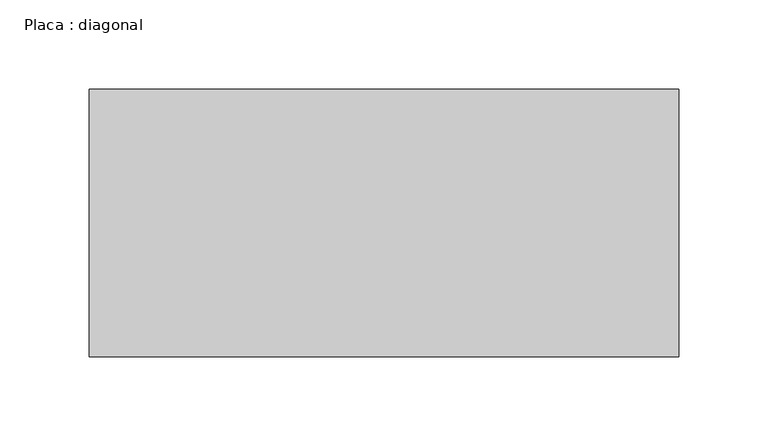
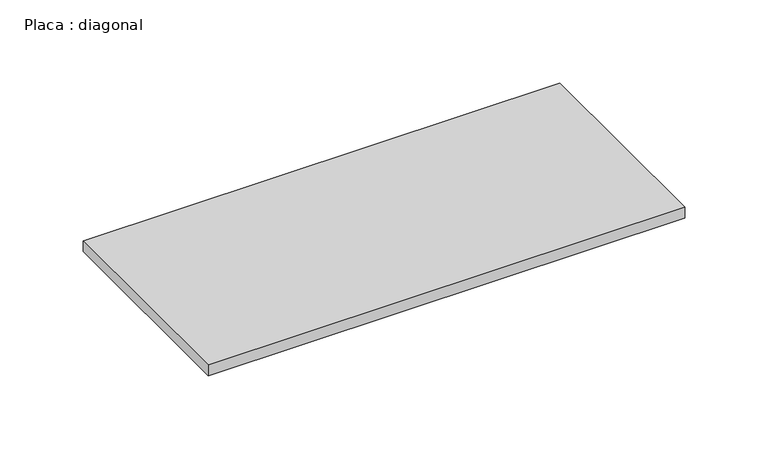
"""IFC4 building model written with IfcOpenShell, lengths in millimetres: beam geometry, Placa : diagonal."""

from ifc_helpers import new_model, si_unit, frame, origin, place, context, project, spatial, polyline, outline, extrude, source, transform, mapped, element, save


def placa_diagonal_af2a04a3(model_context):
    return source(origin(), model_context, "Body", "SweptSolid", [
        extrude(outline(polyline([(165.1705216, 75.0), (165.1705216, -75.0), (-165.4962729, -75.0), (-165.4962729, 75.0), (165.1705216, 75.0)])), frame((0.0, 0.0, -4.0), z_axis=(0.0, 0.0, 1.0), x_axis=(1.0, 0.0, 0.0)), (0.0, 0.0, 1.0), 8.0),
    ])


if __name__ == "__main__":
    model = new_model("IFC4")
    model_context = context("Model", 3, world=origin())
    ifc_project = project(units=[si_unit("LENGTHUNIT", "METRE", prefix="MILLI")], contexts=[model_context])
    site = spatial("IfcSite", under=ifc_project)
    building = spatial("IfcBuilding", under=site)
    placement = place(None, origin())
    placa_diagonal_shape = placa_diagonal_af2a04a3(model_context)
    element("IfcBeam", 1, ObjectType="Placa : diagonal", at=placement, inside=building, context=model_context, shape_type="MappedRepresentation", body=[
        mapped(placa_diagonal_shape, transform((0.0, 0.0, 0.0), x_axis=(1.0, 0.0, 0.0), y_axis=(0.0, 1.0, 0.0), z_axis=(0.0, 0.0, 1.0))),
    ])
    save(model, "model.ifc")

# Revit data of these elements
# Type "Placa : diagonal"
#   W = 0
#   Length [instance default] = 1.50 m
#   b = 0.15 m
#   d = 0.008 m
#   A = 0 m²
#   Structural Material [instance default] = Aço, 45-345
# Element 1 (IfcBeam, "Placa : diagonal")
#   Materials on its faces: "Aço, 45-345"
# Materials
#   "Aço, 45-345": class "Metal", colour RGB 247 247 247, transparency 0, Description = "Aço 345 MPa", Cost = 0
